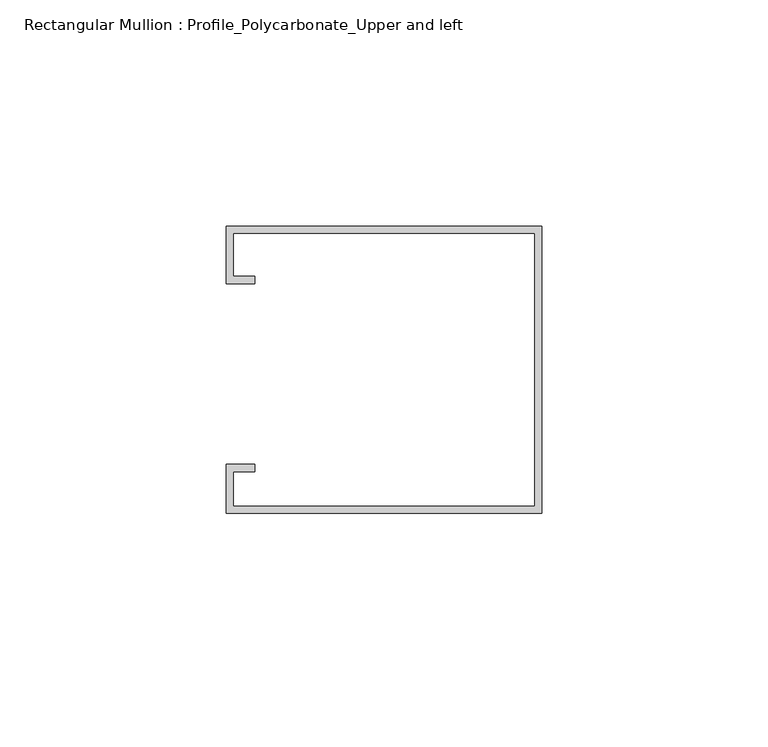
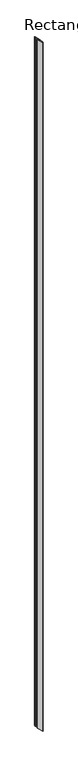
"""IFC4 building model written with IfcOpenShell, lengths in millimetres: member geometry, Rectangular Mullion : Profile_Polycarbonate_Upper and left."""

from ifc_helpers import new_model, si_unit, origin, place, context, project, spatial, faceted_brep, source, transform, mapped, element, save


def rectangular_mullion_profile_polycarbonate_upper_and_left_56d15bf7(model_context):
    return source(origin(), model_context, "Body", "Brep", [
        faceted_brep([(-69.85, 32.7, 64.2712818), (0.0, 32.7, 0.0), (0.0, 32.7, -9315.8792993), (-69.85, 32.7, -9251.6080175), (-69.85, 20.0, 64.2712818), (-69.85, 20.0, -9251.6080175), (-63.5, 20.0, 58.428438), (-63.5, 20.0, -9257.4508613), (-63.5, 21.5875, 58.428438), (-63.5, 21.5875, -9257.4508613), (-68.2625, 21.5875, 62.8105708), (-68.2625, 21.5875, -9253.0687284), (-68.2625, 31.1125, 62.8105708), (-68.2625, 31.1125, -9253.0687284), (-1.5875, 31.1125, 1.4607109), (-1.5875, 31.1125, -9314.4185883), (-1.5875, -29.2125, 1.4607109), (-1.5875, -29.2125, -9314.4185883), (-68.2625, -29.2125, 62.8105708), (-68.2625, -29.2125, -9253.0687284), (-68.2625, -21.5875, 62.8105708), (-68.2625, -21.5875, -9253.0687284), (-63.5, -21.5875, 58.428438), (-63.5, -21.5875, -9257.4508613), (-63.5, -20.0, 58.428438), (-63.5, -20.0, -9257.4508613), (-69.85, -20.0, 64.2712818), (-69.85, -20.0, -9251.6080175), (-69.85, -30.8, 64.2712818), (-69.85, -30.8, -9251.6080175), (0.0, -30.8, 0.0), (0.0, -30.8, -9315.8792993)], [[[0, 1, 2, 3]], [[4, 0, 3, 5]], [[6, 4, 5, 7]], [[8, 6, 7, 9]], [[10, 8, 9, 11]], [[12, 10, 11, 13]], [[14, 12, 13, 15]], [[16, 14, 15, 17]], [[18, 16, 17, 19]], [[20, 18, 19, 21]], [[22, 20, 21, 23]], [[24, 22, 23, 25]], [[26, 24, 25, 27]], [[28, 26, 27, 29]], [[30, 28, 29, 31]], [[1, 30, 31, 2]], [[1, 0, 4, 6, 8, 10, 12, 14, 16, 18, 20, 22, 24, 26, 28, 30]], [[2, 31, 29, 27, 25, 23, 21, 19, 17, 15, 13, 11, 9, 7, 5, 3]]]),
    ])


if __name__ == "__main__":
    model = new_model("IFC4")
    model_context = context("Model", 3, world=origin())
    ifc_project = project(units=[si_unit("LENGTHUNIT", "METRE", prefix="MILLI")], contexts=[model_context])
    site = spatial("IfcSite", under=ifc_project)
    building = spatial("IfcBuilding", under=site)
    placement = place(None, origin())
    rectangular_mullion_profile_polycarbonate_upper_and_left_shape = rectangular_mullion_profile_polycarbonate_upper_and_left_56d15bf7(model_context)
    element("IfcMember", 1, ObjectType="Rectangular Mullion : Profile_Polycarbonate_Upper and left", at=placement, inside=building, context=model_context, shape_type="MappedRepresentation", body=[
        mapped(rectangular_mullion_profile_polycarbonate_upper_and_left_shape, transform((0.0, 0.0, 0.0), x_axis=(1.0, 0.0, 0.0), y_axis=(0.0, 1.0, 0.0), z_axis=(0.0, 0.0, 1.0))),
    ])
    save(model, "model.ifc")

# Revit data of these elements
# Type "Rectangular Mullion : Profile_Polycarbonate_Upper and left"
#   built-in parameter 1007322 = 0.208333 (stored number, unit not read)
#   built-in parameter 1007321 = 0.00520833 (stored number, unit not read)
#   built-in parameter 1007320 = 0 (stored number, unit not read)
# Element 1 (IfcMember, "Rectangular Mullion : Profile_Polycarbonate_Upper and left")
#   Materials on its faces: "ALUMINUM PROFILE AT POLYCARBONATE PANEL"
# Materials
#   "ALUMINUM PROFILE AT POLYCARBONATE PANEL": class "Metal", colour RGB 244 244 244, transparency 0, Description = "Aluminum 6061", Cost = 0
